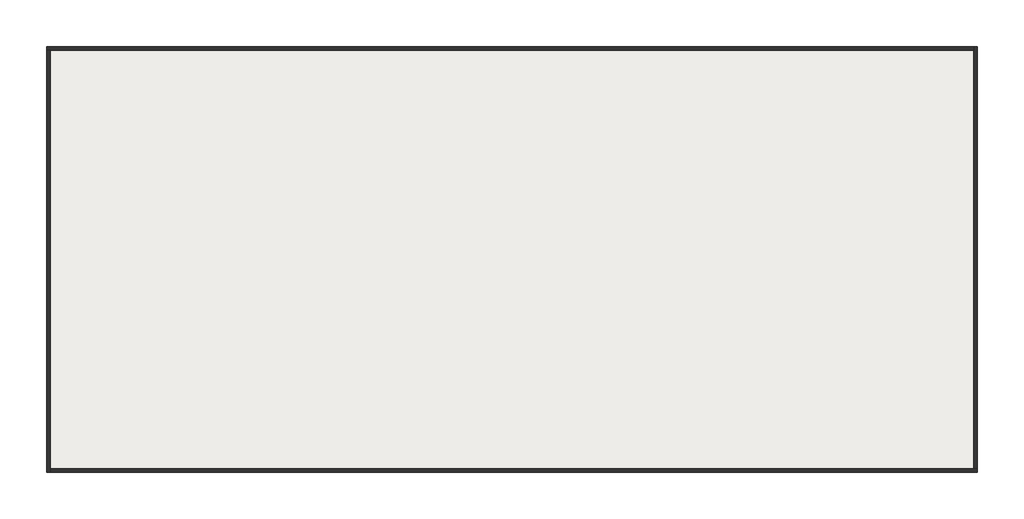
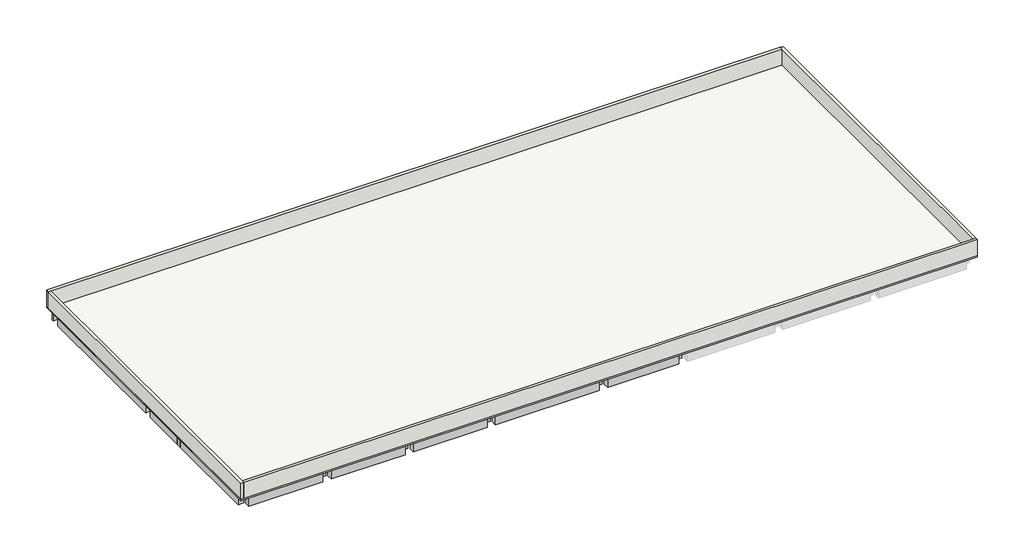
# One storey, part 1 of 2: 29 beams, 4 walls, 1 roof.
"""IFC4 building model written with IfcOpenShell, lengths in millimetres."""

from ifc_helpers import new_model, si_unit, frame, origin, place, context, project, spatial, polyline, outline, extrude, faceted_brep, element, save

model = new_model("IFC4")

# Units and contexts
model_context = context("Model", 3, world=origin())
ifc_project = project(units=[si_unit("LENGTHUNIT", "METRE", prefix="MILLI")], contexts=[model_context])

# Site, building, storey
site = spatial("IfcSite", under=ifc_project)
building = spatial("IfcBuilding", under=site)
storey = spatial("IfcBuildingStorey", under=building, Name="TOC", Elevation=7650.0)

# Beams
placement = place(None, origin())
element("IfcBeam", 1, ObjectType="RC Beam_Rectangular : H_SB_ACB_B400xH900", at=placement, inside=storey, context=model_context, shape_type="Brep", body=[
    faceted_brep([(224.7, 12116.5208589, 7500.0), (224.7, 12116.5208589, 6750.0), (5624.7, 12116.5208589, 6750.0), (5624.7, 12116.5208589, 7500.0), (5724.7, 12116.5208589, 7500.0), (6124.7, 12116.5208589, 7500.0), (6124.7, 12116.5208589, 7549.0), (5724.7, 12116.5208589, 7549.0), (124.7, 12116.5208589, 7549.0), (-275.3, 12116.5208589, 7549.0), (-275.3, 12116.5208589, 7500.0), (124.7, 12116.5208589, 7500.0), (224.7, 12516.5208589, 6750.0), (5624.7, 12516.5208589, 6750.0), (224.7, 12516.5208589, 7500.0), (124.7, 12516.5208589, 7500.0), (-275.3, 12516.5208589, 7500.0), (-275.3, 12516.5208589, 7549.0), (124.7, 12516.5208589, 7549.0), (5724.7, 12516.5208589, 7549.0), (6124.7, 12516.5208589, 7549.0), (6124.7, 12516.5208589, 7500.0), (5724.7, 12516.5208589, 7500.0), (5624.7, 12516.5208589, 7500.0)], [[[0, 1, 2, 3, 4, 5, 6, 7, 8, 9, 10, 11]], [[1, 12, 13, 2]], [[12, 14, 15, 16, 17, 18, 19, 20, 21, 22, 23, 13]], [[1, 0, 14, 12]], [[0, 11, 10, 16, 15, 14]], [[23, 3, 2, 13]], [[3, 23, 22, 21, 5, 4]], [[9, 8, 7, 6, 20, 19, 18, 17]], [[9, 17, 16, 10]], [[20, 6, 5, 21]]]),
])
element("IfcBeam", 2, ObjectType="RC Beam_Rectangular : H_SB_ACB_B400xH900", at=placement, inside=storey, context=model_context, shape_type="Brep", body=[
    faceted_brep([(6224.7, 12116.5208589, 7500.0), (6224.7, 12116.5208589, 6750.0), (11624.7, 12116.5208589, 6750.0), (11624.7, 12116.5208589, 7500.0), (11724.7, 12116.5208589, 7500.0), (12124.7, 12116.5208589, 7500.0), (12124.7, 12116.5208589, 7549.0), (11724.7, 12116.5208589, 7549.0), (6124.7, 12116.5208589, 7549.0), (6124.7, 12116.5208589, 7500.0), (6224.7, 12516.5208589, 6750.0), (11624.7, 12516.5208589, 6750.0), (6224.7, 12516.5208589, 7500.0), (6124.7, 12516.5208589, 7500.0), (6124.7, 12516.5208589, 7549.0), (11724.7, 12516.5208589, 7549.0), (12124.7, 12516.5208589, 7549.0), (12124.7, 12516.5208589, 7500.0), (11724.7, 12516.5208589, 7500.0), (11624.7, 12516.5208589, 7500.0)], [[[0, 1, 2, 3, 4, 5, 6, 7, 8, 9]], [[1, 10, 11, 2]], [[10, 12, 13, 14, 15, 16, 17, 18, 19, 11]], [[1, 0, 12, 10]], [[0, 9, 13, 12]], [[19, 3, 2, 11]], [[3, 19, 18, 17, 5, 4]], [[8, 7, 6, 16, 15, 14]], [[16, 6, 5, 17]], [[8, 14, 13, 9]]]),
])
element("IfcBeam", 3, ObjectType="RC Beam_Rectangular : H_SB_ACB_B400xH900", at=placement, inside=storey, context=model_context, shape_type="Brep", body=[
    faceted_brep([(12224.7, 12116.5208589, 7500.0), (12224.7, 12116.5208589, 6750.0), (17624.7, 12116.5208589, 6750.0), (17624.7, 12116.5208589, 7500.0), (17724.7, 12116.5208589, 7500.0), (18124.7, 12116.5208589, 7500.0), (18124.7, 12116.5208589, 7549.0), (17724.7, 12116.5208589, 7549.0), (12124.7, 12116.5208589, 7549.0), (12124.7, 12116.5208589, 7500.0), (12224.7, 12516.5208589, 6750.0), (17624.7, 12516.5208589, 6750.0), (12224.7, 12516.5208589, 7500.0), (12124.7, 12516.5208589, 7500.0), (12124.7, 12516.5208589, 7549.0), (17724.7, 12516.5208589, 7549.0), (18124.7, 12516.5208589, 7549.0), (18124.7, 12516.5208589, 7500.0), (17724.7, 12516.5208589, 7500.0), (17624.7, 12516.5208589, 7500.0)], [[[0, 1, 2, 3, 4, 5, 6, 7, 8, 9]], [[1, 10, 11, 2]], [[10, 12, 13, 14, 15, 16, 17, 18, 19, 11]], [[1, 0, 12, 10]], [[0, 9, 13, 12]], [[19, 3, 2, 11]], [[3, 19, 18, 17, 5, 4]], [[8, 7, 6, 16, 15, 14]], [[16, 6, 5, 17]], [[8, 14, 13, 9]]]),
])
element("IfcBeam", 4, ObjectType="RC Beam_Rectangular : H_SB_ACB_B400xH900", at=placement, inside=storey, context=model_context, shape_type="Brep", body=[
    faceted_brep([(26324.7, 12116.5208589, 7549.0), (25924.7, 12116.5208589, 7549.0), (18124.7, 12116.5208589, 7549.0), (18124.7, 12116.5208589, 7500.0), (18224.7, 12116.5208589, 7500.0), (18224.7, 12116.5208589, 6750.0), (25924.7, 12116.5208589, 6750.0), (26324.7, 12116.5208589, 6750.0), (26324.7, 12516.5208589, 6750.0), (18224.7, 12516.5208589, 6750.0), (25924.7, 12516.5208589, 6750.0), (18124.7, 12516.5208589, 7549.0), (25924.7, 12516.5208589, 7549.0), (26324.7, 12516.5208589, 7549.0), (18224.7, 12516.5208589, 7500.0), (18124.7, 12516.5208589, 7500.0)], [[[0, 1, 2, 3, 4, 5, 6, 7]], [[8, 7, 6, 5, 9, 10]], [[11, 12, 13, 8, 10, 9, 14, 15]], [[4, 14, 9, 5]], [[14, 4, 3, 15]], [[2, 1, 0, 13, 12, 11]], [[7, 8, 13, 0]], [[2, 11, 15, 3]]]),
])
element("IfcBeam", 5, ObjectType="RC Beam_Rectangular : H_SB_ACB_B400xH900", at=placement, inside=storey, context=model_context, shape_type="Brep", body=[
    faceted_brep([(32124.7, 12116.5208589, 6750.0), (32124.7, 12116.5208589, 7549.0), (31724.7, 12116.5208589, 7549.0), (26324.7, 12116.5208589, 7549.0), (26324.7, 12116.5208589, 6750.0), (31724.7, 12116.5208589, 6750.0), (32124.7, 12516.5208589, 6750.0), (26324.7, 12516.5208589, 6750.0), (31724.7, 12516.5208589, 6750.0), (32124.7, 12516.5208589, 7549.0), (26324.7, 12516.5208589, 7549.0), (31724.7, 12516.5208589, 7549.0)], [[[0, 1, 2, 3, 4, 5]], [[6, 0, 5, 4, 7, 8]], [[9, 6, 8, 7, 10, 11]], [[1, 9, 11, 10, 3, 2]], [[0, 6, 9, 1]], [[4, 3, 10, 7]]]),
])
element("IfcBeam", 6, ObjectType="RC Beam_Rectangular : H_SB_ACB_B400xH900", at=placement, inside=storey, context=model_context, shape_type="Brep", body=[
    faceted_brep([(-275.3, 8216.5208589, 6750.0), (124.7, 8216.5208589, 6750.0), (5724.7, 8216.5208589, 6750.0), (6124.7, 8216.5208589, 6750.0), (6124.7, 8216.5208589, 7549.0), (5724.7, 8216.5208589, 7549.0), (124.7, 8216.5208589, 7549.0), (-275.3, 8216.5208589, 7549.0), (-275.3, 8616.5208589, 6750.0), (124.7, 8616.5208589, 6750.0), (5724.7, 8616.5208589, 6750.0), (6124.7, 8616.5208589, 6750.0), (-275.3, 8616.5208589, 7549.0), (124.7, 8616.5208589, 7549.0), (5724.7, 8616.5208589, 7549.0), (6124.7, 8616.5208589, 7549.0)], [[[0, 1, 2, 3, 4, 5, 6, 7]], [[0, 8, 9, 10, 11, 3, 2, 1]], [[11, 10, 9, 8, 12, 13, 14, 15]], [[7, 6, 5, 4, 15, 14, 13, 12]], [[8, 0, 7, 12]], [[3, 11, 15, 4]]]),
])
element("IfcBeam", 7, ObjectType="RC Beam_Rectangular : H_SB_ACB_B400xH900", at=placement, inside=storey, context=model_context, shape_type="Brep", body=[
    faceted_brep([(12124.7, 8216.5208589, 6750.0), (12124.7, 8216.5208589, 7549.0), (11724.7, 8216.5208589, 7549.0), (6124.7, 8216.5208589, 7549.0), (6124.7, 8216.5208589, 6750.0), (11724.7, 8216.5208589, 6750.0), (12124.7, 8616.5208589, 6750.0), (6124.7, 8616.5208589, 6750.0), (11724.7, 8616.5208589, 6750.0), (12124.7, 8616.5208589, 7549.0), (6124.7, 8616.5208589, 7549.0), (11724.7, 8616.5208589, 7549.0)], [[[0, 1, 2, 3, 4, 5]], [[6, 0, 5, 4, 7, 8]], [[9, 6, 8, 7, 10, 11]], [[1, 9, 11, 10, 3, 2]], [[0, 6, 9, 1]], [[4, 3, 10, 7]]]),
])
element("IfcBeam", 8, ObjectType="RC Beam_Rectangular : H_SB_ACB_B400xH900", at=placement, inside=storey, context=model_context, shape_type="Brep", body=[
    faceted_brep([(18124.7, 8216.5208589, 6750.0), (18124.7, 8216.5208589, 7549.0), (17724.7, 8216.5208589, 7549.0), (12124.7, 8216.5208589, 7549.0), (12124.7, 8216.5208589, 6750.0), (17724.7, 8216.5208589, 6750.0), (18124.7, 8616.5208589, 6750.0), (12124.7, 8616.5208589, 6750.0), (17724.7, 8616.5208589, 6750.0), (18124.7, 8616.5208589, 7549.0), (12124.7, 8616.5208589, 7549.0), (17724.7, 8616.5208589, 7549.0)], [[[0, 1, 2, 3, 4, 5]], [[6, 0, 5, 4, 7, 8]], [[9, 6, 8, 7, 10, 11]], [[1, 9, 11, 10, 3, 2]], [[0, 6, 9, 1]], [[4, 3, 10, 7]]]),
])
element("IfcBeam", 9, ObjectType="RC Beam_Rectangular : H_SB_ACB_B400xH900", at=placement, inside=storey, context=model_context, shape_type="Brep", body=[
    faceted_brep([(26324.7, 8216.5208589, 7549.0), (25924.7, 8216.5208589, 7549.0), (18124.7, 8216.5208589, 7549.0), (18124.7, 8216.5208589, 6750.0), (25824.7, 8216.5208589, 6750.0), (25824.7, 8216.5208589, 7500.0), (25924.7, 8216.5208589, 7500.0), (26324.7, 8216.5208589, 7500.0), (18124.7, 8616.5208589, 6750.0), (25824.7, 8616.5208589, 6750.0), (18124.7, 8616.5208589, 7549.0), (25924.7, 8616.5208589, 7549.0), (26324.7, 8616.5208589, 7549.0), (26324.7, 8616.5208589, 7500.0), (25924.7, 8616.5208589, 7500.0), (25824.7, 8616.5208589, 7500.0)], [[[0, 1, 2, 3, 4, 5, 6, 7]], [[3, 8, 9, 4]], [[10, 11, 12, 13, 14, 15, 9, 8]], [[15, 5, 4, 9]], [[5, 15, 14, 13, 7, 6]], [[2, 1, 0, 12, 11, 10]], [[12, 0, 7, 13]], [[3, 2, 10, 8]]]),
])
element("IfcBeam", 10, ObjectType="RC Beam_Rectangular : H_SB_ACB_B400xH900", at=placement, inside=storey, context=model_context, shape_type="Brep", body=[
    faceted_brep([(26424.7, 8216.5208589, 7500.0), (26424.7, 8216.5208589, 6750.0), (31624.7, 8216.5208589, 6750.0), (31624.7, 8216.5208589, 7500.0), (31724.7, 8216.5208589, 7500.0), (32124.7, 8216.5208589, 7500.0), (32124.7, 8216.5208589, 7549.0), (31724.7, 8216.5208589, 7549.0), (26324.7, 8216.5208589, 7549.0), (26324.7, 8216.5208589, 7500.0), (26424.7, 8616.5208589, 6750.0), (31624.7, 8616.5208589, 6750.0), (26424.7, 8616.5208589, 7500.0), (26324.7, 8616.5208589, 7500.0), (26324.7, 8616.5208589, 7549.0), (31724.7, 8616.5208589, 7549.0), (32124.7, 8616.5208589, 7549.0), (32124.7, 8616.5208589, 7500.0), (31724.7, 8616.5208589, 7500.0), (31624.7, 8616.5208589, 7500.0)], [[[0, 1, 2, 3, 4, 5, 6, 7, 8, 9]], [[1, 10, 11, 2]], [[10, 12, 13, 14, 15, 16, 17, 18, 19, 11]], [[1, 0, 12, 10]], [[0, 9, 13, 12]], [[19, 3, 2, 11]], [[3, 19, 18, 17, 5, 4]], [[8, 7, 6, 16, 15, 14]], [[16, 6, 5, 17]], [[8, 14, 13, 9]]]),
])
element("IfcBeam", 11, ObjectType="RC Beam_Rectangular : H_SB_ACB_B400xH900", at=placement, inside=storey, context=model_context, shape_type="Brep", body=[
    faceted_brep([(224.7, 416.5208589, 7500.0), (224.7, 416.5208589, 6750.0), (5624.7, 416.5208589, 6750.0), (5624.7, 416.5208589, 7500.0), (6124.7, 416.5208589, 7500.0), (6124.7, 416.5208589, 7549.0), (-275.3, 416.5208589, 7549.0), (-275.3, 416.5208589, 7500.0), (224.7, 816.5208589, 6750.0), (5624.7, 816.5208589, 6750.0), (224.7, 816.5208589, 7500.0), (124.7, 816.5208589, 7500.0), (-275.3, 816.5208589, 7500.0), (-275.3, 816.5208589, 7549.0), (124.7, 816.5208589, 7549.0), (5724.7, 816.5208589, 7549.0), (6124.7, 816.5208589, 7549.0), (6124.7, 816.5208589, 7500.0), (5724.7, 816.5208589, 7500.0), (5624.7, 816.5208589, 7500.0)], [[[0, 1, 2, 3, 4, 5, 6, 7]], [[1, 8, 9, 2]], [[8, 10, 11, 12, 13, 14, 15, 16, 17, 18, 19, 9]], [[8, 1, 0, 10]], [[12, 11, 10, 0, 7]], [[19, 3, 2, 9]], [[3, 19, 18, 17, 4]], [[6, 5, 16, 15, 14, 13]], [[6, 13, 12, 7]], [[16, 5, 4, 17]]]),
])
element("IfcBeam", 12, ObjectType="RC Beam_Rectangular : H_SB_ACB_B400xH900", at=placement, inside=storey, context=model_context, shape_type="Brep", body=[
    faceted_brep([(6224.7, 416.5208589, 7500.0), (6224.7, 416.5208589, 6750.0), (11624.7, 416.5208589, 6750.0), (11624.7, 416.5208589, 7500.0), (12124.7, 416.5208589, 7500.0), (12124.7, 416.5208589, 7549.0), (6124.7, 416.5208589, 7549.0), (6124.7, 416.5208589, 7500.0), (6224.7, 816.5208589, 6750.0), (11624.7, 816.5208589, 6750.0), (6224.7, 816.5208589, 7500.0), (6124.7, 816.5208589, 7500.0), (6124.7, 816.5208589, 7549.0), (11724.7, 816.5208589, 7549.0), (12124.7, 816.5208589, 7549.0), (12124.7, 816.5208589, 7500.0), (11724.7, 816.5208589, 7500.0), (11624.7, 816.5208589, 7500.0)], [[[0, 1, 2, 3, 4, 5, 6, 7]], [[1, 8, 9, 2]], [[8, 10, 11, 12, 13, 14, 15, 16, 17, 9]], [[8, 1, 0, 10]], [[11, 10, 0, 7]], [[17, 3, 2, 9]], [[3, 17, 16, 15, 4]], [[6, 5, 14, 13, 12]], [[14, 5, 4, 15]], [[6, 12, 11, 7]]]),
])
element("IfcBeam", 13, ObjectType="RC Beam_Rectangular : H_SB_ACB_B400xH900", at=placement, inside=storey, context=model_context, shape_type="Brep", body=[
    faceted_brep([(12224.7, 416.5208589, 7500.0), (12224.7, 416.5208589, 6750.0), (17624.7, 416.5208589, 6750.0), (17624.7, 416.5208589, 7500.0), (18124.7, 416.5208589, 7500.0), (18124.7, 416.5208589, 7549.0), (12124.7, 416.5208589, 7549.0), (12124.7, 416.5208589, 7500.0), (12224.7, 816.5208589, 6750.0), (17624.7, 816.5208589, 6750.0), (12224.7, 816.5208589, 7500.0), (12124.7, 816.5208589, 7500.0), (12124.7, 816.5208589, 7549.0), (17724.7, 816.5208589, 7549.0), (18124.7, 816.5208589, 7549.0), (18124.7, 816.5208589, 7500.0), (17724.7, 816.5208589, 7500.0), (17624.7, 816.5208589, 7500.0)], [[[0, 1, 2, 3, 4, 5, 6, 7]], [[1, 8, 9, 2]], [[8, 10, 11, 12, 13, 14, 15, 16, 17, 9]], [[8, 1, 0, 10]], [[11, 10, 0, 7]], [[17, 3, 2, 9]], [[3, 17, 16, 15, 4]], [[6, 5, 14, 13, 12]], [[14, 5, 4, 15]], [[6, 12, 11, 7]]]),
])
element("IfcBeam", 14, ObjectType="RC Beam_Rectangular : H_SB_ACB_B400xH900", at=placement, inside=storey, context=model_context, shape_type="Brep", body=[
    faceted_brep([(18224.7, 416.5208589, 7500.0), (18224.7, 416.5208589, 6750.0), (25824.7, 416.5208589, 6750.0), (25824.7, 416.5208589, 7500.0), (26324.7, 416.5208589, 7500.0), (26324.7, 416.5208589, 7549.0), (18124.7, 416.5208589, 7549.0), (18124.7, 416.5208589, 7500.0), (18224.7, 816.5208589, 6750.0), (25824.7, 816.5208589, 6750.0), (18224.7, 816.5208589, 7500.0), (18124.7, 816.5208589, 7500.0), (18124.7, 816.5208589, 7549.0), (25924.7, 816.5208589, 7549.0), (26324.7, 816.5208589, 7549.0), (26324.7, 816.5208589, 7500.0), (25924.7, 816.5208589, 7500.0), (25824.7, 816.5208589, 7500.0)], [[[0, 1, 2, 3, 4, 5, 6, 7]], [[1, 8, 9, 2]], [[8, 10, 11, 12, 13, 14, 15, 16, 17, 9]], [[8, 1, 0, 10]], [[11, 10, 0, 7]], [[17, 3, 2, 9]], [[3, 17, 16, 15, 4]], [[6, 5, 14, 13, 12]], [[14, 5, 4, 15]], [[6, 12, 11, 7]]]),
])
element("IfcBeam", 15, ObjectType="RC Beam_Rectangular : H_SB_ACB_B400xH900", at=placement, inside=storey, context=model_context, shape_type="Brep", body=[
    faceted_brep([(26424.7, 416.5208589, 7500.0), (26424.7, 416.5208589, 6750.0), (31624.7, 416.5208589, 6750.0), (31624.7, 416.5208589, 7500.0), (32124.7, 416.5208589, 7500.0), (32124.7, 416.5208589, 7549.0), (26324.7, 416.5208589, 7549.0), (26324.7, 416.5208589, 7500.0), (26424.7, 816.5208589, 6750.0), (31624.7, 816.5208589, 6750.0), (26424.7, 816.5208589, 7500.0), (26324.7, 816.5208589, 7500.0), (26324.7, 816.5208589, 7549.0), (31724.7, 816.5208589, 7549.0), (32124.7, 816.5208589, 7549.0), (32124.7, 816.5208589, 7500.0), (31724.7, 816.5208589, 7500.0), (31624.7, 816.5208589, 7500.0)], [[[0, 1, 2, 3, 4, 5, 6, 7]], [[1, 8, 9, 2]], [[8, 10, 11, 12, 13, 14, 15, 16, 17, 9]], [[8, 1, 0, 10]], [[11, 10, 0, 7]], [[17, 3, 2, 9]], [[3, 17, 16, 15, 4]], [[6, 5, 14, 13, 12]], [[14, 5, 4, 15]], [[6, 12, 11, 7]]]),
])
element("IfcBeam", 16, ObjectType="RC Beam_Rectangular : H_SB_ACB_B400xH900", at=placement, inside=storey, context=model_context, shape_type="SweptSolid", body=[
    extrude(outline(polyline([(8216.5208589, 7549.0), (8216.5208589, 6750.0), (916.5208589, 6750.0), (916.5208589, 7500.0), (816.5208589, 7500.0), (816.5208589, 7549.0), (8216.5208589, 7549.0)])), frame((-275.3, 0.0, 0.0), z_axis=(1.0, 0.0, 0.0), x_axis=(0.0, 1.0, 0.0)), (0.0, 0.0, 1.0), 400.0),
])
element("IfcBeam", 17, ObjectType="RC Beam_Rectangular : H_SB_ACB_B400xH900", at=placement, inside=storey, context=model_context, shape_type="SweptSolid", body=[
    extrude(outline(polyline([(8616.5208589, 7549.0), (12116.5208589, 7549.0), (12116.5208589, 7500.0), (12016.5208589, 7500.0), (12016.5208589, 6750.0), (8616.5208589, 6750.0), (8616.5208589, 7549.0)])), frame((-275.3, 0.0, 0.0), z_axis=(1.0, 0.0, 0.0), x_axis=(0.0, 1.0, 0.0)), (0.0, 0.0, 1.0), 400.0),
])
element("IfcBeam", 18, ObjectType="RC Beam_Rectangular : H_SB_ACB_B400xH900", at=placement, inside=storey, context=model_context, shape_type="Brep", body=[
    faceted_brep([(124.7, 24429.2208589, 6750.0), (-275.3, 24429.2208589, 6750.0), (-275.3, 24429.2208589, 7549.0), (124.7, 24429.2208589, 7549.0), (124.7, 12616.5208589, 7500.0), (124.7, 12616.5208589, 6750.0), (124.7, 23716.5208589, 6750.0), (124.7, 23716.5208589, 7500.0), (124.7, 23816.5208589, 7500.0), (124.7, 24216.5208589, 7500.0), (124.7, 24316.5208589, 7500.0), (124.7, 24316.5208589, 6750.0), (124.7, 24216.5208589, 7549.0), (124.7, 23816.5208589, 7549.0), (124.7, 12516.5208589, 7549.0), (124.7, 12516.5208589, 7500.0), (-275.3, 24316.5208589, 6750.0), (-275.3, 12616.5208589, 6750.0), (-275.3, 12616.5208589, 7500.0), (-275.3, 12516.5208589, 7500.0), (-275.3, 12516.5208589, 7549.0), (-275.3, 24316.5208589, 7500.0), (-275.3, 23716.5208589, 7500.0), (-275.3, 23716.5208589, 6750.0)], [[[0, 1, 2, 3]], [[4, 5, 6, 7, 8, 9, 10, 11, 0, 3, 12, 13, 14, 15]], [[1, 0, 11, 16]], [[17, 18, 19, 20, 2, 1, 16, 21, 22, 23]], [[19, 15, 14, 20]], [[5, 4, 18, 17]], [[4, 15, 19, 18]], [[22, 7, 6, 23]], [[7, 22, 21, 10, 9, 8]], [[3, 2, 20, 14, 13, 12]], [[10, 21, 16, 11]], [[5, 17, 23, 6]]]),
])
element("IfcBeam", 19, ObjectType="RC Beam_Rectangular : H_SB_ACB_B400xH900", at=placement, inside=storey, context=model_context, shape_type="SweptSolid", body=[
    extrude(outline(polyline([(8216.5208589, 7549.0), (8216.5208589, 6750.0), (916.5208589, 6750.0), (916.5208589, 7500.0), (816.5208589, 7500.0), (816.5208589, 7549.0), (8216.5208589, 7549.0)])), frame((5724.7, 0.0, 0.0), z_axis=(1.0, 0.0, 0.0), x_axis=(0.0, 1.0, 0.0)), (0.0, 0.0, 1.0), 400.0),
])
element("IfcBeam", 20, ObjectType="RC Beam_Rectangular : H_SB_ACB_B400xH900", at=placement, inside=storey, context=model_context, shape_type="SweptSolid", body=[
    extrude(outline(polyline([(8616.5208589, 6750.0), (8616.5208589, 7549.0), (12116.5208589, 7549.0), (12116.5208589, 7500.0), (12016.5208589, 7500.0), (12016.5208589, 6750.0), (8616.5208589, 6750.0)])), frame((5724.7, 0.0, 0.0), z_axis=(1.0, 0.0, 0.0), x_axis=(0.0, 1.0, 0.0)), (0.0, 0.0, 1.0), 400.0),
])
element("IfcBeam", 21, ObjectType="RC Beam_Rectangular : H_SB_ACB_B400xH900", at=placement, inside=storey, context=model_context, shape_type="Brep", body=[
    faceted_brep([(6124.7, 24429.2208589, 6750.0), (5724.7, 24429.2208589, 6750.0), (5724.7, 24429.2208589, 7549.0), (6124.7, 24429.2208589, 7549.0), (6124.7, 12616.5208589, 7500.0), (6124.7, 12616.5208589, 6750.0), (6124.7, 23716.5208589, 6750.0), (6124.7, 23716.5208589, 7500.0), (6124.7, 23816.5208589, 7500.0), (6124.7, 24216.5208589, 7500.0), (6124.7, 24316.5208589, 7500.0), (6124.7, 24316.5208589, 6750.0), (6124.7, 24216.5208589, 7549.0), (6124.7, 23816.5208589, 7549.0), (6124.7, 12516.5208589, 7549.0), (6124.7, 12516.5208589, 7500.0), (5724.7, 24316.5208589, 6750.0), (5724.7, 24316.5208589, 7500.0), (5724.7, 24216.5208589, 7500.0), (5724.7, 23816.5208589, 7500.0), (5724.7, 23716.5208589, 7500.0), (5724.7, 23716.5208589, 6750.0), (5724.7, 12616.5208589, 6750.0), (5724.7, 12616.5208589, 7500.0), (5724.7, 12516.5208589, 7500.0), (5724.7, 12516.5208589, 7549.0), (5724.7, 23816.5208589, 7549.0), (5724.7, 24216.5208589, 7549.0)], [[[0, 1, 2, 3]], [[4, 5, 6, 7, 8, 9, 10, 11, 0, 3, 12, 13, 14, 15]], [[1, 0, 11, 16]], [[2, 1, 16, 17, 18, 19, 20, 21, 22, 23, 24, 25, 26, 27]], [[24, 15, 14, 25]], [[5, 4, 23, 22]], [[4, 15, 24, 23]], [[20, 7, 6, 21]], [[7, 20, 19, 18, 17, 10, 9, 8]], [[3, 2, 27, 26, 25, 14, 13, 12]], [[10, 17, 16, 11]], [[5, 22, 21, 6]]]),
])
element("IfcBeam", 22, ObjectType="RC Beam_Rectangular : H_SB_ACB_B400xH900", at=placement, inside=storey, context=model_context, shape_type="SweptSolid", body=[
    extrude(outline(polyline([(8216.5208589, 7549.0), (8216.5208589, 6750.0), (916.5208589, 6750.0), (916.5208589, 7500.0), (816.5208589, 7500.0), (816.5208589, 7549.0), (8216.5208589, 7549.0)])), frame((11724.7, 0.0, 0.0), z_axis=(1.0, 0.0, 0.0), x_axis=(0.0, 1.0, 0.0)), (0.0, 0.0, 1.0), 400.0),
])
element("IfcBeam", 23, ObjectType="RC Beam_Rectangular : H_SB_ACB_B400xH900", at=placement, inside=storey, context=model_context, shape_type="SweptSolid", body=[
    extrude(outline(polyline([(8616.5208589, 6750.0), (8616.5208589, 7549.0), (12116.5208589, 7549.0), (12116.5208589, 7500.0), (12016.5208589, 7500.0), (12016.5208589, 6750.0), (8616.5208589, 6750.0)])), frame((11724.7, 0.0, 0.0), z_axis=(1.0, 0.0, 0.0), x_axis=(0.0, 1.0, 0.0)), (0.0, 0.0, 1.0), 400.0),
])
element("IfcBeam", 24, ObjectType="RC Beam_Rectangular : H_SB_ACB_B400xH900", at=placement, inside=storey, context=model_context, shape_type="SweptSolid", body=[
    extrude(outline(polyline([(8216.5208589, 7549.0), (8216.5208589, 6750.0), (916.5208589, 6750.0), (916.5208589, 7500.0), (816.5208589, 7500.0), (816.5208589, 7549.0), (8216.5208589, 7549.0)])), frame((17724.7, 0.0, 0.0), z_axis=(1.0, 0.0, 0.0), x_axis=(0.0, 1.0, 0.0)), (0.0, 0.0, 1.0), 400.0),
])
element("IfcBeam", 25, ObjectType="RC Beam_Rectangular : H_SB_ACB_B400xH900", at=placement, inside=storey, context=model_context, shape_type="SweptSolid", body=[
    extrude(outline(polyline([(8616.5208589, 6750.0), (8616.5208589, 7549.0), (12116.5208589, 7549.0), (12116.5208589, 7500.0), (12016.5208589, 7500.0), (12016.5208589, 6750.0), (8616.5208589, 6750.0)])), frame((17724.7, 0.0, 0.0), z_axis=(1.0, 0.0, 0.0), x_axis=(0.0, 1.0, 0.0)), (0.0, 0.0, 1.0), 400.0),
])
element("IfcBeam", 26, ObjectType="RC Beam_Rectangular : H_SB_ACB_B400xH900", at=placement, inside=storey, context=model_context, shape_type="SweptSolid", body=[
    extrude(outline(polyline([(8116.5208589, 7500.0), (8116.5208589, 6750.0), (916.5208589, 6750.0), (916.5208589, 7500.0), (816.5208589, 7500.0), (816.5208589, 7549.0), (8216.5208589, 7549.0), (8216.5208589, 7500.0), (8116.5208589, 7500.0)])), frame((25924.7, 0.0, 0.0), z_axis=(1.0, 0.0, 0.0), x_axis=(0.0, 1.0, 0.0)), (0.0, 0.0, 1.0), 400.0),
])
element("IfcBeam", 27, ObjectType="RC Beam_Rectangular : H_SB_ACB_B400xH900", at=placement, inside=storey, context=model_context, shape_type="SweptSolid", body=[
    extrude(outline(polyline([(12116.5208589, 7549.0), (12116.5208589, 6750.0), (8716.5208589, 6750.0), (8716.5208589, 7500.0), (8616.5208589, 7500.0), (8616.5208589, 7549.0), (12116.5208589, 7549.0)])), frame((25924.7, 0.0, 0.0), z_axis=(1.0, 0.0, 0.0), x_axis=(0.0, 1.0, 0.0)), (0.0, 0.0, 1.0), 400.0),
])
element("IfcBeam", 28, ObjectType="RC Beam_Rectangular : H_SB_ACB_B400xH900", at=placement, inside=storey, context=model_context, shape_type="SweptSolid", body=[
    extrude(outline(polyline([(8116.5208589, 7500.0), (8116.5208589, 6750.0), (916.5208589, 6750.0), (916.5208589, 7500.0), (816.5208589, 7500.0), (816.5208589, 7549.0), (8216.5208589, 7549.0), (8216.5208589, 7500.0), (8116.5208589, 7500.0)])), frame((31724.7, 0.0, 0.0), z_axis=(1.0, 0.0, 0.0), x_axis=(0.0, 1.0, 0.0)), (0.0, 0.0, 1.0), 400.0),
])
element("IfcBeam", 29, ObjectType="RC Beam_Rectangular : H_SB_ACB_B400xH900", at=placement, inside=storey, context=model_context, shape_type="SweptSolid", body=[
    extrude(outline(polyline([(12116.5208589, 7549.0), (12116.5208589, 6750.0), (8716.5208589, 6750.0), (8716.5208589, 7500.0), (8616.5208589, 7500.0), (8616.5208589, 7549.0), (12116.5208589, 7549.0)])), frame((31724.7, 0.0, 0.0), z_axis=(1.0, 0.0, 0.0), x_axis=(0.0, 1.0, 0.0)), (0.0, 0.0, 1.0), 400.0),
])

# Roof
element("IfcRoof", 30, ObjectType="H_RF_AMF_RC Roof Finish_WP_Insulation_Protection", at=placement, inside=storey, context=model_context, shape_type="SweptSolid", body=[
    extrude(outline(polyline([(53324.7, 24816.5208589), (53324.7, 216.5208589), (-475.3, 216.5208589), (-475.3, 24816.5208589), (53324.7, 24816.5208589)])), frame((0.0, 0.0, 7549.0), z_axis=(0.0, 0.0, 1.0), x_axis=(1.0, 0.0, 0.0)), (0.0, 0.0, 1.0), 101.0),
])

# Walls
element("IfcWall", 31, ObjectType="H_WA_AMW_RC Wall_T200 (No Finish)", at=placement, inside=storey, context=model_context, shape_type="Brep", body=[
    faceted_brep([(-475.3, 24616.5208589, 7650.0), (-275.3, 24616.5208589, 7650.0), (53124.7, 24616.5208589, 7650.0), (53124.7, 24616.5208589, 8900.0), (-275.3, 24616.5208589, 8900.0), (-475.3, 24616.5208589, 8900.0), (-475.3, 24816.5208589, 7650.0), (-475.3, 24816.5208589, 8900.0), (53124.7, 24816.5208589, 8900.0), (53124.7, 24816.5208589, 7650.0)], [[[0, 1, 2, 3, 4, 5]], [[6, 7, 8, 9]], [[2, 1, 0, 6, 9]], [[5, 4, 3, 8, 7]], [[0, 5, 7, 6]], [[3, 2, 9, 8]]]),
])
element("IfcWall", 32, ObjectType="H_WA_AMW_RC Wall_T200 (No Finish)", at=placement, inside=storey, context=model_context, shape_type="Brep", body=[
    faceted_brep([(-275.3, 216.5208589, 7650.0), (-275.3, 416.5208589, 7650.0), (-275.3, 24616.5208589, 7650.0), (-275.3, 24616.5208589, 8900.0), (-275.3, 416.5208589, 8900.0), (-275.3, 216.5208589, 8900.0), (-475.3, 216.5208589, 7650.0), (-475.3, 216.5208589, 8900.0), (-475.3, 24616.5208589, 8900.0), (-475.3, 24616.5208589, 7650.0)], [[[0, 1, 2, 3, 4, 5]], [[6, 7, 8, 9]], [[2, 1, 0, 6, 9]], [[5, 4, 3, 8, 7]], [[0, 5, 7, 6]], [[3, 2, 9, 8]]]),
])
element("IfcWall", 33, ObjectType="H_WA_AMW_RC Wall_T200 (No Finish)", at=placement, inside=storey, context=model_context, shape_type="Brep", body=[
    faceted_brep([(53324.7, 416.5208589, 7650.0), (53124.7, 416.5208589, 7650.0), (-275.3, 416.5208589, 7650.0), (-275.3, 416.5208589, 8900.0), (53124.7, 416.5208589, 8900.0), (53324.7, 416.5208589, 8900.0), (53324.7, 216.5208589, 7650.0), (53324.7, 216.5208589, 8900.0), (-275.3, 216.5208589, 8900.0), (-275.3, 216.5208589, 7650.0)], [[[0, 1, 2, 3, 4, 5]], [[6, 7, 8, 9]], [[2, 1, 0, 6, 9]], [[5, 4, 3, 8, 7]], [[0, 5, 7, 6]], [[3, 2, 9, 8]]]),
])
element("IfcWall", 34, ObjectType="H_WA_AMW_RC Wall_T200 (No Finish)", at=placement, inside=storey, context=model_context, shape_type="Brep", body=[
    faceted_brep([(53124.7, 24816.5208589, 7650.0), (53124.7, 24616.5208589, 7650.0), (53124.7, 416.5208589, 7650.0), (53124.7, 416.5208589, 8900.0), (53124.7, 24616.5208589, 8900.0), (53124.7, 24816.5208589, 8900.0), (53324.7, 24816.5208589, 7650.0), (53324.7, 24816.5208589, 8900.0), (53324.7, 416.5208589, 8900.0), (53324.7, 416.5208589, 7650.0)], [[[0, 1, 2, 3, 4, 5]], [[6, 7, 8, 9]], [[2, 1, 0, 6, 9]], [[5, 4, 3, 8, 7]], [[0, 5, 7, 6]], [[3, 2, 9, 8]]]),
])

save(model, "model.ifc")

# Revit data of these elements
# Type "RC Beam_Rectangular : H_SB_ACB_B400xH900"
#   중앙부 하부근 = ""
#   중앙부 상부근 = ""
#   중앙부 보조근 = ""
#   중앙부 늑근 = ""
#   외단부 하부근 = ""
#   외단부 상부근 = ""
#   외단부 보조근 = ""
#   외단부 늑근 = ""
#   부호 = "TG3"
#   내단부 하부근 = ""
#   내단부 상부근 = ""
#   내단부 보조근 = ""
#   내단부 늑근 = ""
#   ALL 하부근 = "3-D20"
#   ALL 상부근 = "3-D20"
#   ALL 보조근 = ""
#   ALL 늑근 = "2-D10 @120"
#   Width = 400.000 mm
#   Height = 900.000 mm
#   Length [instance default] = 1524.000 mm
#   b = 400.000 mm
#   h = 900.000 mm
#   hec_material3 [instance default] = none
#   hec_material2 [instance default] = none
#   hec_material1 [instance default] = none
#   Structural Material [instance default] = none
#   Assembly Code = ""
# Type "H_RF_AMF_RC Roof Finish_WP_Insulation_Protection"
#   Layers, outside or top first: 50.000 mm no material (function 4); 0.000 mm no material (function 100); 50.000 mm no material (function 3); 1.000 mm no material (function 2)
# Type "H_WA_AMW_RC Wall_T200 (No Finish)"
#   Type Comments = ""
#   Layers, outside or top first: 0.000 mm no material (function 100); 0.000 mm no material (function 100); 200.000 mm no material (function 1); 0.000 mm no material (function 100); 0.000 mm no material (function 100); 0.000 mm no material (function 100)
# Elements 1, 2, 3, 4, 5, 6, 7, 8, 9, 10, 11, 12, 13, 14, 15, 16, 17, 18, 19, 20, 21, 22, 23, 24, 25, 26, 27, 28, 29 (IfcBeam, "RC Beam_Rectangular : H_SB_ACB_B400xH900")
#   hec_material3 = none
#   hec_material2 = none
#   hec_material1 = none
#   Structural Material = none
#   Phase Created = New Construction
# Element 30 (IfcRoof, "H_RF_AMF_RC Roof Finish_WP_Insulation_Protection")
#   Mark = "RF1"
#   Roof Style Name = "Lightweight Concrete(Slope)+Insulation+Waterproofing+Gravel"
#   Roof Ref. = ""
#   Roof Base Material = "Concrete Slab"
#   Roof Finish_1 = "Light-Weight Concrete Screed (Slope 1%)"
#   Roof Finish_2 = ""
#   Roof Finish_3 = "Rigid Extruded Polystyrene Foam Insulation(XPS)"
#   Roof Finish_4 = "Waterproofing Membrane-EPDM(or Equivalent)"
#   Roof Finish_5 = "Gravel for Roof"
#   built-in parameter 1001705 = 25.0984 (stored number, unit not read)
#   built-in parameter 1001701 = -0.331365 (stored number, unit not read)
#   built-in parameter 1001710 = 33615
#   Roof Style = RF13
#   Phase Created = New Construction
#   Materials on its faces: "Default Roof"
# Element 31 (IfcWall, "H_WA_AMW_RC Wall_T200 (No Finish)")
#   Mark = "PW1"
#   Wall Loca = "ROOF"
#   Wall Style Name = "Concrete Wall+Acrylic Emulsion Paint on Cement Plaster"
#   Wall Ref. = ""
#   Wall Finish-In = ""
#   Wall Base Material-1 = ""
#   Wall Base Material-2 = ""
#   Wall Base Material-3 = "Concrete Wall"
#   Wall Finish-Ex = "Acrylic Emulsion Paint on Fair Faced Concrete"
#   Top Offset = 0.000 mm
#   Base Offset = 0.000 mm
#   wall height = 1250.000 mm
#   Wall Style No = EW51
#   Phase Created = New Construction
#   Base Constraint = TOC
#   Top Constraint = TOP
#   Materials on its faces: "Default Wall"
# Element 32 (IfcWall, "H_WA_AMW_RC Wall_T200 (No Finish)")
#   Mark = "PW2"
#   Wall Loca = "ROOF"
#   Wall Style Name = "Concrete Wall+Acrylic Emulsion Paint on Cement Plaster"
#   Wall Ref. = ""
#   Wall Finish-In = ""
#   Wall Base Material-1 = ""
#   Wall Base Material-2 = ""
#   Wall Base Material-3 = "Concrete Wall"
#   Wall Finish-Ex = "Acrylic Emulsion Paint on Fair Faced Concrete"
#   Top Offset = 0.000 mm
#   Base Offset = 0.000 mm
#   wall height = 1250.000 mm
#   Wall Style No = EW51
#   Phase Created = New Construction
#   Base Constraint = TOC
#   Top Constraint = TOP
#   Materials on its faces: "Default Wall"
# Element 33 (IfcWall, "H_WA_AMW_RC Wall_T200 (No Finish)")
#   Mark = "PW3"
#   Wall Loca = "ROOF"
#   Wall Style Name = "Concrete Wall+Acrylic Emulsion Paint on Cement Plaster"
#   Wall Ref. = ""
#   Wall Finish-In = ""
#   Wall Base Material-1 = ""
#   Wall Base Material-2 = ""
#   Wall Base Material-3 = "Concrete Wall"
#   Wall Finish-Ex = "Acrylic Emulsion Paint on Fair Faced Concrete"
#   Top Offset = 0.000 mm
#   Base Offset = 0.000 mm
#   wall height = 1250.000 mm
#   Wall Style No = EW51
#   Phase Created = New Construction
#   Base Constraint = TOC
#   Top Constraint = TOP
#   Materials on its faces: "Default Wall"
# Element 34 (IfcWall, "H_WA_AMW_RC Wall_T200 (No Finish)")
#   Mark = "PW4"
#   Wall Loca = "ROOF"
#   Wall Style Name = "Concrete Wall+Acrylic Emulsion Paint on Cement Plaster"
#   Wall Ref. = ""
#   Wall Finish-In = ""
#   Wall Base Material-1 = ""
#   Wall Base Material-2 = ""
#   Wall Base Material-3 = "Concrete Wall"
#   Wall Finish-Ex = "Acrylic Emulsion Paint on Fair Faced Concrete"
#   Top Offset = 0.000 mm
#   Base Offset = 0.000 mm
#   wall height = 1250.000 mm
#   Wall Style No = EW51
#   Phase Created = New Construction
#   Base Constraint = TOC
#   Top Constraint = TOP
#   Materials on its faces: "Default Wall"
# Materials
#   "Default Roof": class "Miscellaneous", colour RGB 80 80 80, transparency 0
#   "Default Wall": class "Miscellaneous", colour RGB 80 80 80, transparency 0
# Room at (24679.385, 12577.526) mm, phase "New Construction", upper level "TOC", upper offset 2000.000 mm, lower offset 0.000 mm
#   Comments = ""
#   Number = "129"
#   Name = "ROOF"
